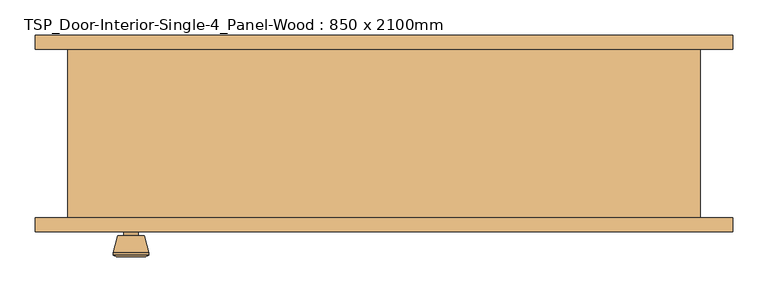
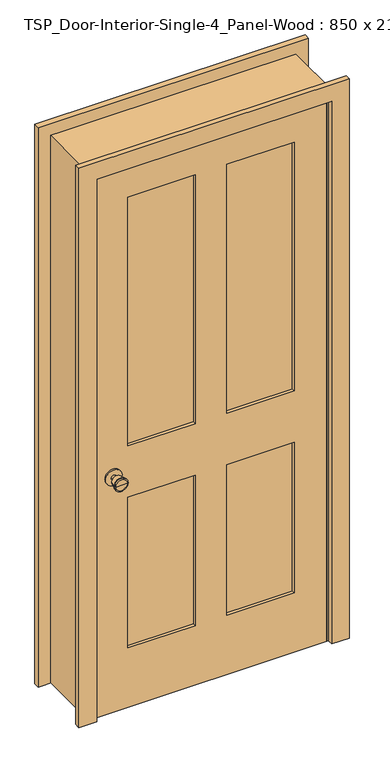
"""IFC4 building model written with IfcOpenShell, lengths in millimetres: door geometry, TSP_Door-Interior-Single-4_Panel-Wood : 850 x 2100mm."""

from ifc_helpers import new_model, si_unit, point, frame, frame_2d, origin, place, context, project, spatial, polyline, circle_curve, trimmed, segment, composite_curve, outline, extrude, faceted_brep, source, transform, mapped, element, save
from ifc_brep_helpers import plane_surface, cylinder_surface, revolved_surface, advanced_brep


def tsp_door_interior_single_4_panel_wood_850_x_2100mm_e1b314b4(model_context):
    return source(origin(), model_context, "Body", "SolidModel", [
        advanced_brep(
        [(-360.0, -75.825, 914.4), (-370.0, -75.825, 914.4), (-350.0, -75.825, 914.4), (-339.5241324, -26.825, 914.4), (-380.4758676, -26.825, 914.4), (-360.0, -26.825, 914.4), (-335.0, -28.6528681, 914.4), (-385.0, -28.6528681, 914.4), (-335.0, -32.1165463, 914.4), (-385.0, -32.1165463, 914.4), (-341.363764, -56.825, 914.4), (-378.636236, -56.825, 914.4), (-350.0, -56.825, 914.4), (-370.0, -56.825, 914.4)],
        [
            (0, 1),
            (1, 2, circle_curve(frame((-360.0, -75.825, 914.4), z_axis=(0.0, -1.0, 0.0), x_axis=(-1.0, 0.0, 0.0)), 10.0)),
            (2, 0),
            (2, 1, circle_curve(frame((-360.0, -75.825, 914.4), z_axis=(0.0, -1.0, 0.0), x_axis=(-1.0, 0.0, 0.0)), 10.0)),
            (3, 4, circle_curve(frame((-360.0, -26.825, 914.4), z_axis=(0.0, 1.0, 0.0), x_axis=(-1.0, 0.0, 0.0)), 20.4758676)),
            (4, 5),
            (5, 3),
            (4, 3, circle_curve(frame((-360.0, -26.825, 914.4), z_axis=(0.0, 1.0, 0.0), x_axis=(-1.0, 0.0, 0.0)), 20.4758676)),
            (6, 7, circle_curve(frame((-360.0, -28.6528681, 914.4), z_axis=(0.0, 1.0, 0.0), x_axis=(-1.0, 0.0, 0.0)), 25.0)),
            (7, 4),
            (3, 6),
            (7, 6, circle_curve(frame((-360.0, -28.6528681, 914.4), z_axis=(0.0, 1.0, 0.0), x_axis=(-1.0, 0.0, 0.0)), 25.0)),
            (8, 9, circle_curve(frame((-360.0, -32.1165463, 914.4), z_axis=(0.0, 1.0, 0.0), x_axis=(-1.0, 0.0, 0.0)), 25.0)),
            (9, 7),
            (6, 8),
            (9, 8, circle_curve(frame((-360.0, -32.1165463, 914.4), z_axis=(0.0, 1.0, 0.0), x_axis=(-1.0, 0.0, 0.0)), 25.0)),
            (10, 11, circle_curve(frame((-360.0, -56.825, 914.4), z_axis=(0.0, 1.0, 0.0), x_axis=(-1.0, 0.0, 0.0)), 18.636236)),
            (11, 9),
            (8, 10),
            (11, 10, circle_curve(frame((-360.0, -56.825, 914.4), z_axis=(0.0, 1.0, 0.0), x_axis=(-1.0, 0.0, 0.0)), 18.636236)),
            (12, 13, circle_curve(frame((-360.0, -56.825, 914.4), z_axis=(0.0, 1.0, 0.0), x_axis=(-1.0, 0.0, 0.0)), 10.0)),
            (13, 11),
            (10, 12),
            (13, 12, circle_curve(frame((-360.0, -56.825, 914.4), z_axis=(0.0, 1.0, 0.0), x_axis=(-1.0, 0.0, 0.0)), 10.0)),
            (1, 13),
            (12, 2),
        ],
        [
            plane_surface(frame((-360.0, -75.825, 914.4), z_axis=(0.0, -1.0, 0.0), x_axis=(-1.0, 0.0, 0.0))),
            plane_surface(frame((-360.0, -26.825, 914.4), z_axis=(0.0, 1.0, 0.0), x_axis=(-1.0, 0.0, 0.0))),
            revolved_surface(polyline([(-380.4758676, -26.825, 914.4), (-385.0, -28.6528681, 914.4)]), (-360.0, -75.825, 914.4), (0.0, -1.0, 0.0)),
            cylinder_surface(frame((-360.0, -75.825, 914.4), z_axis=(0.0, -1.0, 0.0), x_axis=(-1.0, 0.0, 0.0)), 25.0),
            revolved_surface(polyline([(-385.0, -32.1165463, 914.4), (-378.636236, -56.825, 914.4)]), (-360.0, -75.825, 914.4), (0.0, -1.0, 0.0)),
            plane_surface(frame((-360.0, -56.825, 914.4), z_axis=(0.0, -1.0, 0.0), x_axis=(-1.0, 0.0, 0.0))),
            cylinder_surface(frame((-360.0, -75.825, 914.4), z_axis=(0.0, -1.0, 0.0), x_axis=(-1.0, 0.0, 0.0)), 10.0),
        ],
        [
            (0, [[1, 2, 3]]),
            (0, [[-3, 4, -1]]),
            (1, [[5, 6, 7]]),
            (1, [[8, -7, -6]]),
            (2, [[9, 10, -5, 11]]),
            (2, [[12, -11, -8, -10]]),
            (3, [[13, 14, -9, 15]]),
            (3, [[16, -15, -12, -14]]),
            (4, [[17, 18, -13, 19]]),
            (4, [[20, -19, -16, -18]]),
            (5, [[21, 22, -17, 23]]),
            (5, [[24, -23, -20, -22]]),
            (6, [[-2, 25, -21, 26]]),
            (6, [[-4, -26, -24, -25]]),
        ],
    ),
        extrude(outline(composite_curve([segment(trimmed(circle_curve(frame_2d((914.4, -360.0)), 30.0), [point((914.4, -390.0))], [point((914.4, -330.0))], False, "CARTESIAN"), True, "CONTINUOUS"), segment(trimmed(circle_curve(frame_2d((914.4, -360.0)), 30.0), [point((914.4, -330.0))], [point((914.4, -390.0))], False, "CARTESIAN"), True, "CONTINUOUS")], self_intersect=False)), frame((0.0, -81.825, 0.0), z_axis=(0.0, 1.0, 0.0), x_axis=(0.0, 0.0, 1.0)), (0.0, 0.0, 1.0), 6.0),
        advanced_brep(
        [(-360.0, -122.825, 914.4), (-350.0, -122.825, 914.4), (-370.0, -122.825, 914.4), (-339.5241324, -171.825, 914.4), (-360.0, -171.825, 914.4), (-380.4758676, -171.825, 914.4), (-335.0, -169.9971319, 914.4), (-385.0, -169.9971319, 914.4), (-335.0, -166.5334537, 914.4), (-385.0, -166.5334537, 914.4), (-341.363764, -141.825, 914.4), (-378.636236, -141.825, 914.4), (-350.0, -141.825, 914.4), (-370.0, -141.825, 914.4)],
        [
            (0, 1),
            (1, 2, circle_curve(frame((-360.0, -122.825, 914.4), z_axis=(0.0, 1.0, 0.0), x_axis=(-1.0, 0.0, 0.0)), 10.0)),
            (2, 0),
            (2, 1, circle_curve(frame((-360.0, -122.825, 914.4), z_axis=(0.0, 1.0, 0.0), x_axis=(-1.0, 0.0, 0.0)), 10.0)),
            (3, 4),
            (4, 5),
            (5, 3, circle_curve(frame((-360.0, -171.825, 914.4), z_axis=(0.0, -1.0, 0.0), x_axis=(-1.0, 0.0, 0.0)), 20.4758676)),
            (3, 5, circle_curve(frame((-360.0, -171.825, 914.4), z_axis=(0.0, -1.0, 0.0), x_axis=(-1.0, 0.0, 0.0)), 20.4758676)),
            (6, 3),
            (5, 7),
            (7, 6, circle_curve(frame((-360.0, -169.9971319, 914.4), z_axis=(0.0, -1.0, 0.0), x_axis=(-1.0, 0.0, 0.0)), 25.0)),
            (6, 7, circle_curve(frame((-360.0, -169.9971319, 914.4), z_axis=(0.0, -1.0, 0.0), x_axis=(-1.0, 0.0, 0.0)), 25.0)),
            (8, 6),
            (7, 9),
            (9, 8, circle_curve(frame((-360.0, -166.5334537, 914.4), z_axis=(0.0, -1.0, 0.0), x_axis=(-1.0, 0.0, 0.0)), 25.0)),
            (8, 9, circle_curve(frame((-360.0, -166.5334537, 914.4), z_axis=(0.0, -1.0, 0.0), x_axis=(-1.0, 0.0, 0.0)), 25.0)),
            (10, 8),
            (9, 11),
            (11, 10, circle_curve(frame((-360.0, -141.825, 914.4), z_axis=(0.0, -1.0, 0.0), x_axis=(-1.0, 0.0, 0.0)), 18.636236)),
            (10, 11, circle_curve(frame((-360.0, -141.825, 914.4), z_axis=(0.0, -1.0, 0.0), x_axis=(-1.0, 0.0, 0.0)), 18.636236)),
            (12, 10),
            (11, 13),
            (13, 12, circle_curve(frame((-360.0, -141.825, 914.4), z_axis=(0.0, -1.0, 0.0), x_axis=(-1.0, 0.0, 0.0)), 10.0)),
            (12, 13, circle_curve(frame((-360.0, -141.825, 914.4), z_axis=(0.0, -1.0, 0.0), x_axis=(-1.0, 0.0, 0.0)), 10.0)),
            (1, 12),
            (13, 2),
        ],
        [
            plane_surface(frame((-360.0, -122.825, 914.4), z_axis=(0.0, 1.0, 0.0), x_axis=(-1.0, 0.0, 0.0))),
            plane_surface(frame((-360.0, -171.825, 914.4), z_axis=(0.0, -1.0, 0.0), x_axis=(-1.0, 0.0, 0.0))),
            revolved_surface(polyline([(-380.4758676, -171.825, 914.4), (-385.0, -169.9971319, 914.4)]), (-360.0, -122.825, 914.4), (0.0, 1.0, 0.0)),
            cylinder_surface(frame((-360.0, -122.825, 914.4), z_axis=(0.0, 1.0, 0.0), x_axis=(-1.0, 0.0, 0.0)), 25.0),
            revolved_surface(polyline([(-385.0, -166.5334537, 914.4), (-378.636236, -141.825, 914.4)]), (-360.0, -122.825, 914.4), (0.0, 1.0, 0.0)),
            plane_surface(frame((-360.0, -141.825, 914.4), z_axis=(0.0, 1.0, 0.0), x_axis=(-1.0, 0.0, 0.0))),
            cylinder_surface(frame((-360.0, -122.825, 914.4), z_axis=(0.0, 1.0, 0.0), x_axis=(-1.0, 0.0, 0.0)), 10.0),
        ],
        [
            (0, [[1, 2, 3]]),
            (0, [[-3, 4, -1]]),
            (1, [[5, 6, 7]]),
            (1, [[-6, -5, 8]]),
            (2, [[9, -7, 10, 11]]),
            (2, [[-10, -8, -9, 12]]),
            (3, [[13, -11, 14, 15]]),
            (3, [[-14, -12, -13, 16]]),
            (4, [[17, -15, 18, 19]]),
            (4, [[-18, -16, -17, 20]]),
            (5, [[21, -19, 22, 23]]),
            (5, [[-22, -20, -21, 24]]),
            (6, [[25, -23, 26, -2]]),
            (6, [[-26, -24, -25, -4]]),
        ],
    ),
        extrude(outline(composite_curve([segment(trimmed(circle_curve(frame_2d((914.4, -360.0)), 30.0), [point((914.4, -390.0))], [point((914.4, -330.0))], False, "CARTESIAN"), True, "CONTINUOUS"), segment(trimmed(circle_curve(frame_2d((914.4, -360.0)), 30.0), [point((914.4, -330.0))], [point((914.4, -390.0))], False, "CARTESIAN"), True, "CONTINUOUS")], self_intersect=False)), frame((0.0, -122.825, 0.0), z_axis=(0.0, 1.0, 0.0), x_axis=(0.0, 0.0, 1.0)), (0.0, 0.0, 1.0), 6.0),
        faceted_brep([(450.0, -116.825, 0.0), (425.0, -116.825, 0.0), (425.0, -81.825, 0.0), (412.3, -81.825, 0.0), (412.3, -46.9, 0.0), (425.0, -46.9, 0.0), (425.0, 123.175, 0.0), (450.0, 123.175, 0.0), (450.0, 123.175, 2125.0), (450.0, -116.825, 2125.0), (425.0, 123.175, 2100.0), (-425.0, 123.175, 2100.0), (-425.0, 123.175, 0.0), (-450.0, 123.175, 0.0), (-450.0, 123.175, 2125.0), (425.0, -46.9, 2100.0), (412.3, -46.9, 2087.3), (-412.3, -46.9, 2087.3), (-412.3, -46.9, 0.0), (-425.0, -46.9, 0.0), (-425.0, -46.9, 2100.0), (412.3, -81.825, 2087.3), (425.0, -81.825, 2100.0), (-425.0, -81.825, 2100.0), (-425.0, -81.825, 0.0), (-412.3, -81.825, 0.0), (-412.3, -81.825, 2087.3), (425.0, -116.825, 2100.0), (-450.0, -116.825, 2125.0), (-450.0, -116.825, 0.0), (-425.0, -116.825, 0.0), (-425.0, -116.825, 2100.0)], [[[0, 1, 2, 3, 4, 5, 6, 7]], [[7, 8, 9, 0]], [[6, 10, 11, 12, 13, 14, 8, 7]], [[5, 15, 10, 6]], [[4, 16, 17, 18, 19, 20, 15, 5]], [[3, 21, 16, 4]], [[2, 22, 23, 24, 25, 26, 21, 3]], [[1, 27, 22, 2]], [[0, 9, 28, 29, 30, 31, 27, 1]], [[8, 14, 28, 9]], [[15, 20, 11, 10]], [[21, 26, 17, 16]], [[27, 31, 23, 22]], [[29, 13, 12, 19, 18, 25, 24, 30]], [[14, 13, 29, 28]], [[20, 19, 12, 11]], [[26, 25, 18, 17]], [[31, 30, 24, 23]]]),
        extrude(outline(polyline([(2100.0, -425.0), (0.0, -425.0), (0.0, 425.0), (2100.0, 425.0), (2100.0, -425.0)]), holes=[polyline([(1980.0, 57.5), (1980.0, 305.0), (1014.4, 305.0), (1014.4, 57.5), (1980.0, 57.5)]), polyline([(1014.4, -57.5), (1014.4, -305.0), (1980.0, -305.0), (1980.0, -57.5), (1014.4, -57.5)]), polyline([(814.4, 57.5), (814.4, 305.0), (230.0, 305.0), (230.0, 57.5), (814.4, 57.5)]), polyline([(230.0, -57.5), (230.0, -305.0), (814.4, -305.0), (814.4, -57.5), (230.0, -57.5)])]), frame((0.0, -116.825, 0.0), z_axis=(0.0, 1.0, 0.0), x_axis=(0.0, 0.0, 1.0)), (0.0, 0.0, 1.0), 35.0),
        extrude(outline(polyline([(305.0, -93.4916667), (305.0, -105.1583333), (57.5, -105.1583333), (57.5, -93.4916667), (305.0, -93.4916667)])), frame((0.0, 0.0, 1014.4), z_axis=(0.0, 0.0, 1.0), x_axis=(1.0, 0.0, 0.0)), (0.0, 0.0, 1.0), 965.6),
        extrude(outline(polyline([(-57.5, -93.4916667), (-57.5, -105.1583333), (-305.0, -105.1583333), (-305.0, -93.4916667), (-57.5, -93.4916667)])), frame((0.0, 0.0, 1014.4), z_axis=(0.0, 0.0, 1.0), x_axis=(1.0, 0.0, 0.0)), (0.0, 0.0, 1.0), 965.6),
        extrude(outline(polyline([(305.0, -93.4916667), (305.0, -105.1583333), (57.5, -105.1583333), (57.5, -93.4916667), (305.0, -93.4916667)])), frame((0.0, 0.0, 230.0), z_axis=(0.0, 0.0, 1.0), x_axis=(1.0, 0.0, 0.0)), (0.0, 0.0, 1.0), 584.4),
        extrude(outline(polyline([(-57.5, -93.4916667), (-57.5, -105.1583333), (-305.0, -105.1583333), (-305.0, -93.4916667), (-57.5, -93.4916667)])), frame((0.0, 0.0, 230.0), z_axis=(0.0, 0.0, 1.0), x_axis=(1.0, 0.0, 0.0)), (0.0, 0.0, 1.0), 584.4),
        extrude(outline(polyline([(0.0, 496.35), (2171.35, 496.35), (2171.35, -496.35), (0.0, -496.35), (0.0, -431.35), (2106.35, -431.35), (2106.35, 431.35), (0.0, 431.35), (0.0, 496.35)])), frame((0.0, -136.825, 0.0), z_axis=(0.0, 1.0, 0.0), x_axis=(0.0, 0.0, 1.0)), (0.0, 0.0, 1.0), 20.0),
        extrude(outline(polyline([(0.0, 496.35), (2171.35, 496.35), (2171.35, -496.35), (0.0, -496.35), (0.0, -431.35), (2106.35, -431.35), (2106.35, 431.35), (0.0, 431.35), (0.0, 496.35)])), frame((0.0, 123.175, 0.0), z_axis=(0.0, 1.0, 0.0), x_axis=(0.0, 0.0, 1.0)), (0.0, 0.0, 1.0), 20.0),
    ])


if __name__ == "__main__":
    model = new_model("IFC4")
    model_context = context("Model", 3, world=origin())
    ifc_project = project(units=[si_unit("LENGTHUNIT", "METRE", prefix="MILLI")], contexts=[model_context])
    site = spatial("IfcSite", under=ifc_project)
    building = spatial("IfcBuilding", under=site)
    placement = place(None, origin())
    tsp_door_interior_single_4_panel_wood_850_x_2100mm_shape = tsp_door_interior_single_4_panel_wood_850_x_2100mm_e1b314b4(model_context)
    element("IfcDoor", 1, ObjectType="TSP_Door-Interior-Single-4_Panel-Wood : 850 x 2100mm", at=placement, inside=building, context=model_context, shape_type="MappedRepresentation", body=[
        mapped(tsp_door_interior_single_4_panel_wood_850_x_2100mm_shape, transform((0.0, 0.0, 0.0), x_axis=(1.0, 0.0, 0.0), y_axis=(0.0, 1.0, 0.0), z_axis=(0.0, 0.0, 1.0))),
    ])
    save(model, "model.ifc")

# Revit data of these elements
# Type "TSP_Door-Interior-Single-4_Panel-Wood : 850 x 2100mm"
#   Model = "TSP_DOOR02W"
#   Type Mark = "243"
#   Assembly Code = "C1020300"
#   Analytic Construction = "Wooden"
#   Top Rail = 120 mm
#   Thickness = 35 mm
#   Thermal Resistance (R) = 0.455703 (m²·K)/W
#   Swing Angle [instance default] = 90.00°
#   Stiles = 120 mm
#   Rough Width = 900 mm
#   Rough Height = 2125 mm
#   Mullion = 115 mm
#   Lock Rail = 200 mm
#   Height = 2100 mm
#   Width = 850 mm
#   Heat Transfer Coefficient (U) = 2.19465 W/(m²·K)
#   Bottom Rail = 230 mm
#   Define Thermal Properties by = 1
#   Trim Material = Cherry
#   Panel Material = Cherry
#   Frame Material = Cherry
#   Door Handle Material = Aluminum
#   Visual Light Transmittance = 0
#   Solar Heat Gain Coefficient = 0
#   Wall Closure = (empty or 0)
#   Function = (empty or 0)
# Element 1 (IfcDoor, "TSP_Door-Interior-Single-4_Panel-Wood : 850 x 2100mm")
#   Materials on its faces: "Cherry", "Aluminum"
# Materials
#   "Cherry": class "Wood", colour RGB 226 177 128, transparency 0, Description = "Prunus Serotina", Cost = 0
#   "Aluminum": class "Metal", colour RGB 247 247 247, transparency 0, Description = "Aluminum 6061", Cost = 0
